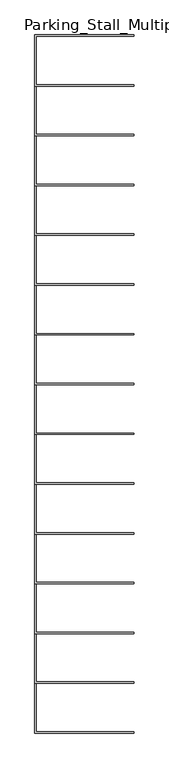
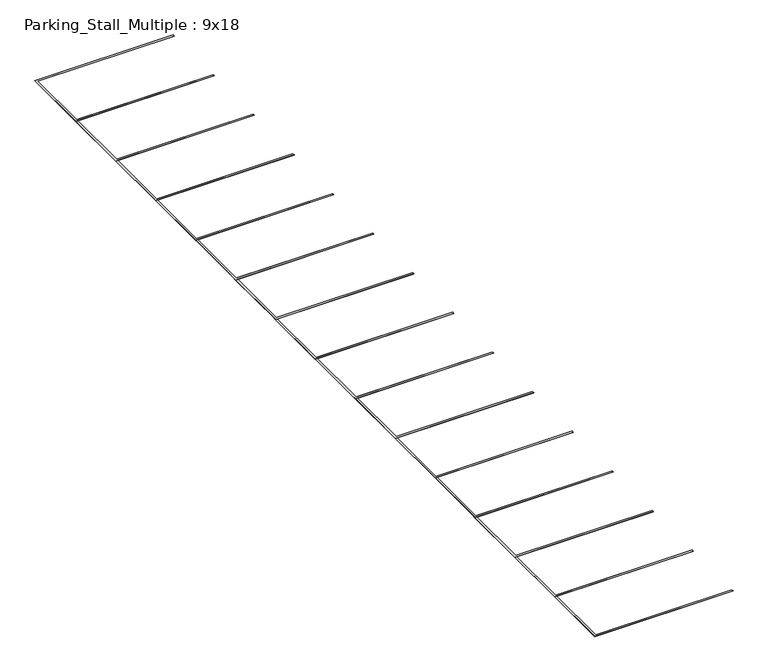
"""IFC4 building model written with IfcOpenShell, lengths in millimetres: proxy geometry, Parking_Stall_Multiple : 9x18."""

from ifc_helpers import new_model, si_unit, origin, origin_with_axes, place, context, project, spatial, polyline, outline, extrude, source, transform, mapped, element, save


def parking_stall_multiple_9x18_4ba3b90c(model_context):
    return source(origin(), model_context, "Body", "SweptSolid", [
        extrude(outline(polyline([(5486.4, 35661.6), (0.0, 35661.6), (0.0, 38481.0), (5486.4, 38481.0), (5486.4, 38404.8), (76.2, 38404.8), (76.2, 35737.8), (5486.4, 35737.8), (5486.4, 35661.6)])), origin_with_axes(), (0.0, 0.0, 1.0), 6.35),
        extrude(outline(polyline([(5486.4, 32918.4), (0.0, 32918.4), (0.0, 35737.8), (5486.4, 35737.8), (5486.4, 35661.6), (76.2, 35661.6), (76.2, 32994.6), (5486.4, 32994.6), (5486.4, 32918.4)])), origin_with_axes(), (0.0, 0.0, 1.0), 6.35),
        extrude(outline(polyline([(5486.4, 30175.2), (0.0, 30175.2), (0.0, 32994.6), (5486.4, 32994.6), (5486.4, 32918.4), (76.2, 32918.4), (76.2, 30251.4), (5486.4, 30251.4), (5486.4, 30175.2)])), origin_with_axes(), (0.0, 0.0, 1.0), 6.35),
        extrude(outline(polyline([(5486.4, 27432.0), (0.0, 27432.0), (0.0, 30251.4), (5486.4, 30251.4), (5486.4, 30175.2), (76.2, 30175.2), (76.2, 27508.2), (5486.4, 27508.2), (5486.4, 27432.0)])), origin_with_axes(), (0.0, 0.0, 1.0), 6.35),
        extrude(outline(polyline([(5486.4, 24688.8), (0.0, 24688.8), (0.0, 27508.2), (5486.4, 27508.2), (5486.4, 27432.0), (76.2, 27432.0), (76.2, 24765.0), (5486.4, 24765.0), (5486.4, 24688.8)])), origin_with_axes(), (0.0, 0.0, 1.0), 6.35),
        extrude(outline(polyline([(5486.4, 21945.6), (0.0, 21945.6), (0.0, 24765.0), (5486.4, 24765.0), (5486.4, 24688.8), (76.2, 24688.8), (76.2, 22021.8), (5486.4, 22021.8), (5486.4, 21945.6)])), origin_with_axes(), (0.0, 0.0, 1.0), 6.35),
        extrude(outline(polyline([(5486.4, 19202.4), (0.0, 19202.4), (0.0, 22021.8), (5486.4, 22021.8), (5486.4, 21945.6), (76.2, 21945.6), (76.2, 19278.6), (5486.4, 19278.6), (5486.4, 19202.4)])), origin_with_axes(), (0.0, 0.0, 1.0), 6.35),
        extrude(outline(polyline([(5486.4, 16459.2), (0.0, 16459.2), (0.0, 19278.6), (5486.4, 19278.6), (5486.4, 19202.4), (76.2, 19202.4), (76.2, 16535.4), (5486.4, 16535.4), (5486.4, 16459.2)])), origin_with_axes(), (0.0, 0.0, 1.0), 6.35),
        extrude(outline(polyline([(5486.4, 13716.0), (0.0, 13716.0), (0.0, 16535.4), (5486.4, 16535.4), (5486.4, 16459.2), (76.2, 16459.2), (76.2, 13792.2), (5486.4, 13792.2), (5486.4, 13716.0)])), origin_with_axes(), (0.0, 0.0, 1.0), 6.35),
        extrude(outline(polyline([(5486.4, 10972.8), (0.0, 10972.8), (0.0, 13792.2), (5486.4, 13792.2), (5486.4, 13716.0), (76.2, 13716.0), (76.2, 11049.0), (5486.4, 11049.0), (5486.4, 10972.8)])), origin_with_axes(), (0.0, 0.0, 1.0), 6.35),
        extrude(outline(polyline([(5486.4, 8229.6), (0.0, 8229.6), (0.0, 11049.0), (5486.4, 11049.0), (5486.4, 10972.8), (76.2, 10972.8), (76.2, 8305.8), (5486.4, 8305.8), (5486.4, 8229.6)])), origin_with_axes(), (0.0, 0.0, 1.0), 6.35),
        extrude(outline(polyline([(5486.4, 5486.4), (0.0, 5486.4), (0.0, 8305.8), (5486.4, 8305.8), (5486.4, 8229.6), (76.2, 8229.6), (76.2, 5562.6), (5486.4, 5562.6), (5486.4, 5486.4)])), origin_with_axes(), (0.0, 0.0, 1.0), 6.35),
        extrude(outline(polyline([(5486.4, 2743.2), (0.0, 2743.2), (0.0, 5562.6), (5486.4, 5562.6), (5486.4, 5486.4), (76.2, 5486.4), (76.2, 2819.4), (5486.4, 2819.4), (5486.4, 2743.2)])), origin_with_axes(), (0.0, 0.0, 1.0), 6.35),
        extrude(outline(polyline([(5486.4, 0.0), (0.0, 0.0), (0.0, 2819.4), (5486.4, 2819.4), (5486.4, 2743.2), (76.2, 2743.2), (76.2, 76.2), (5486.4, 76.2), (5486.4, 0.0)])), origin_with_axes(), (0.0, 0.0, 1.0), 6.35),
    ])


if __name__ == "__main__":
    model = new_model("IFC4")
    model_context = context("Model", 3, world=origin())
    ifc_project = project(units=[si_unit("LENGTHUNIT", "METRE", prefix="MILLI")], contexts=[model_context])
    site = spatial("IfcSite", under=ifc_project)
    building = spatial("IfcBuilding", under=site)
    placement = place(None, origin())
    parking_stall_multiple_9x18_shape = parking_stall_multiple_9x18_4ba3b90c(model_context)
    element("IfcBuildingElementProxy", 1, Name="Parking_Stall_Multiple : 9x18", ObjectType="Parking_Stall_Multiple : 9x18", at=placement, inside=building, context=model_context, shape_type="MappedRepresentation", body=[
        mapped(parking_stall_multiple_9x18_shape, transform((0.0, 0.0, 0.0), x_axis=(1.0, 0.0, 0.0), y_axis=(0.0, 1.0, 0.0), z_axis=(0.0, 0.0, 1.0))),
    ])
    save(model, "model.ifc")

# Revit data of these elements
# Type "Parking_Stall_Multiple : 9x18"
#   Parking_Width_M = 9' - 0"
#   Parking_Run_Length [instance default] = 65' - 0"
#   Parking_Line_Width = 0' - 3"
#   Parking_Length_M = 18' - 0"
#   Single_Parking_Visibility [instance default] = no
#   Parking_ADA_Symbol = no
#   ParkingUnitsArray [instance default] = 7
#   ParkingUnits [instance default] = 7
#   Multiple_Parking_Visibility [instance default] = yes
#   Parking_Line_Material = none
# Element 1 (IfcBuildingElementProxy, "Parking_Stall_Multiple : 9x18")
#   Parking_Run_Length = 124' - 4.95431"
#   ParkingUnitsArray = 14
#   ParkingUnits = 14
